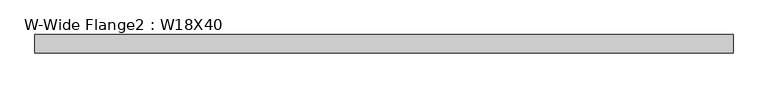
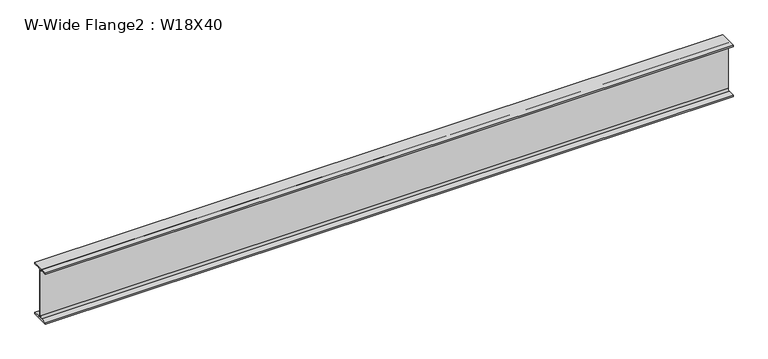
"""IFC4 building model written with IfcOpenShell, lengths in millimetres: beam geometry, W-Wide Flange2 : W18X40."""

from ifc_helpers import new_model, si_unit, point, frame, frame_2d, origin, place, context, project, spatial, polyline, circle_curve, trimmed, segment, composite_curve, outline, extrude, source, transform, mapped, element, save


def w_wide_flange2_w18x40_a80abbf0(model_context):
    return source(origin(), model_context, "Body", "SweptSolid", [
        extrude(outline(composite_curve([segment(polyline([(76.454, -213.995), (76.454, -227.33), (-76.454, -227.33), (-76.454, -213.995), (-20.828, -213.995)]), True, "CONTINUOUS"), segment(trimmed(circle_curve(frame_2d((-20.828, -197.1675)), 16.8275), [point((-20.828, -213.995))], [point((-4.0005, -197.1675))], True, "CARTESIAN"), True, "CONTINUOUS"), segment(polyline([(-4.0005, -197.1675), (-4.0005, 197.1675)]), True, "CONTINUOUS"), segment(trimmed(circle_curve(frame_2d((-20.828, 197.1675)), 16.8275), [point((-4.0005, 197.1675))], [point((-20.828, 213.995))], True, "CARTESIAN"), True, "CONTINUOUS"), segment(polyline([(-20.828, 213.995), (-76.454, 213.995), (-76.454, 227.33), (76.454, 227.33), (76.454, 213.995), (20.828, 213.995)]), True, "CONTINUOUS"), segment(trimmed(circle_curve(frame_2d((20.828, 197.1675)), 16.8275), [point((20.828, 213.995))], [point((4.0005, 197.1675))], True, "CARTESIAN"), True, "CONTINUOUS"), segment(polyline([(4.0005, 197.1675), (4.0005, -197.1675)]), True, "CONTINUOUS"), segment(trimmed(circle_curve(frame_2d((20.828, -197.1675)), 16.8275), [point((4.0005, -197.1675))], [point((20.828, -213.995))], True, "CARTESIAN"), True, "CONTINUOUS"), segment(polyline([(20.828, -213.995), (76.454, -213.995)]), True, "CONTINUOUS")], self_intersect=False)), frame((-2876.153125, 0.0, 0.0), z_axis=(1.0, 0.0, 0.0), x_axis=(0.0, 1.0, 0.0)), (0.0, 0.0, 1.0), 5752.30625),
    ])


if __name__ == "__main__":
    model = new_model("IFC4")
    model_context = context("Model", 3, world=origin())
    ifc_project = project(units=[si_unit("LENGTHUNIT", "METRE", prefix="MILLI")], contexts=[model_context])
    site = spatial("IfcSite", under=ifc_project)
    building = spatial("IfcBuilding", under=site)
    placement = place(None, origin())
    w_wide_flange2_w18x40_shape = w_wide_flange2_w18x40_a80abbf0(model_context)
    element("IfcBeam", 1, ObjectType="W-Wide Flange2 : W18X40", at=placement, inside=building, context=model_context, shape_type="MappedRepresentation", body=[
        mapped(w_wide_flange2_w18x40_shape, transform((0.0, 0.0, 0.0), x_axis=(1.0, 0.0, 0.0), y_axis=(0.0, 1.0, 0.0), z_axis=(0.0, 0.0, 1.0))),
    ])
    save(model, "model.ifc")

# Revit data of these elements
# Type "W-Wide Flange2 : W18X40"
#   Assembly Code = "B10"
#   W = 40
#   Length [instance default] = 5' - 0"
#   bf = 0' - 6.02"
#   d = 1' - 5.9"
#   k = 0' - 1 3/16"
#   k2 = 0' - 0.6625"
#   tf = 0' - 0.525"
#   tw = 0' - 0.315"
#   A = 0.0819444 SF
#   Structural Material [instance default] = Steel ASTM A992
# Element 1 (IfcBeam, "W-Wide Flange2 : W18X40")
#   Materials on its faces: "Steel ASTM A992"
# Materials
#   "Steel ASTM A992": class "Metal", colour RGB 199 199 199, transparency 0, Description = "Structural steel 50ksi", Cost = 0
